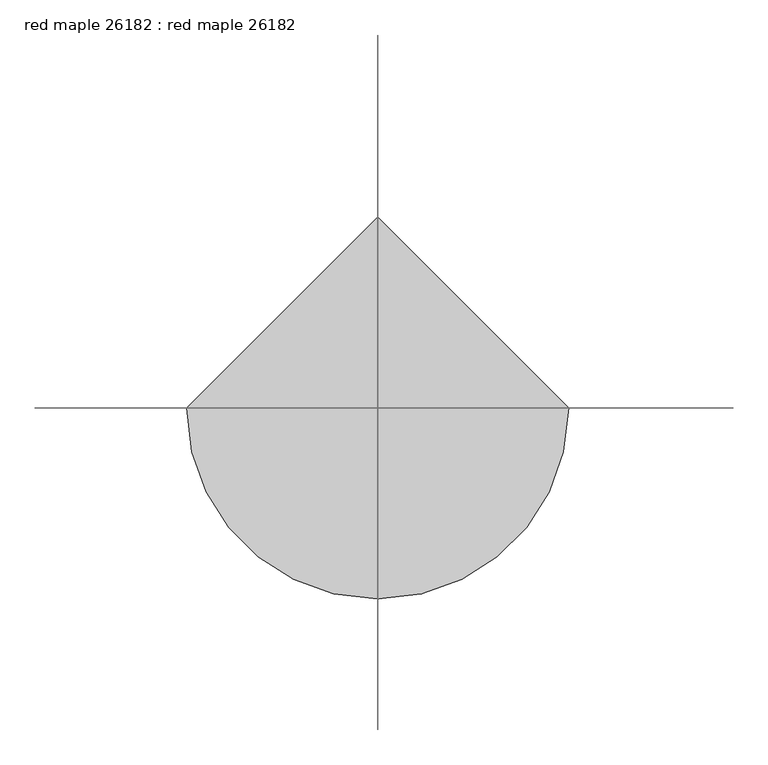
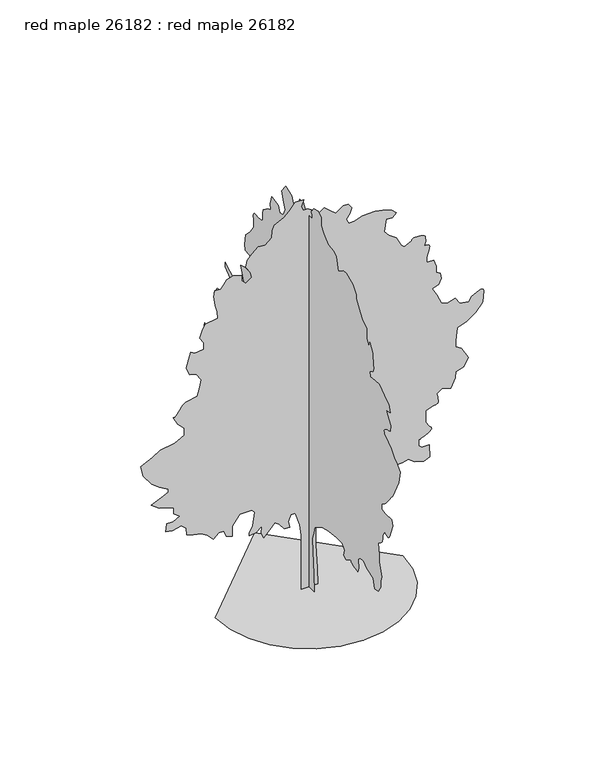
"""IFC4 building model written with IfcOpenShell, lengths in millimetres: proxy geometry, red maple 26182 : red maple 26182."""

from ifc_helpers import new_model, si_unit, origin, place, context, project, spatial, triangles, source, transform, mapped, element, save


def red_maple_26182_red_maple_26182_cba750cc(model_context):
    return source(origin(), model_context, "Body", "Tessellation", [
        triangles([(5.9e-06, 200.5240248, 0.0131599), (5.9e-06, -200.5423013, 0.0131599), (5.9e-06, -173.8047255, 401.079007), (5.9e-06, -147.0663684, 922.4677488), (5.9e-06, -133.6980892, 1216.5822092), (5.9e-06, -173.8047255, 1363.6407475), (5.9e-06, -227.2806583, 1537.4352264), (5.9e-06, -320.8632274, 1590.9124855), (5.9e-06, -534.7644153, 1711.2323215), (5.9e-06, -762.0361897, 1764.7071098), (5.9e-06, -1069.5212002, 1804.8136734), (5.9e-06, -1283.4223881, 1804.8136734), (5.9e-06, -1377.0037399, 1697.8617714), (5.9e-06, -1336.897031, 1550.8033058), (5.9e-06, -1443.848933, 1510.6967422), (5.9e-06, -1617.6460281, 1604.2805649), (5.9e-06, -1620.762553, 1592.8200726), (5.9e-06, -1625.400642, 1581.362051), (5.9e-06, -1633.0790977, 1569.9041748), (5.9e-06, -1645.319339, 1558.4436825), (5.9e-06, -1663.6378429, 1546.9856609), (5.9e-06, -1689.5560284, 1535.5251686), (5.9e-06, -1724.595314, 1524.0672924), (5.9e-06, -1761.1942429, 1514.1662979), (5.9e-06, -1791.4812023, 1507.0721088), (5.9e-06, -1816.5027855, 1502.3197826), (5.9e-06, -1837.3156139, 1499.4343483), (5.9e-06, -1854.971077, 1497.9534794), (5.9e-06, -1870.5234707, 1497.4074371), (5.9e-06, -1885.021859, 1497.3286629), (5.9e-06, -1911.7604885, 1590.9124855), (5.9e-06, -1898.3924091, 1791.445594), (5.9e-06, -1978.6056816, 1871.6588665), (5.9e-06, -2112.293597, 1885.0269459), (5.9e-06, -2219.245499, 1778.0750439), (5.9e-06, -2473.2533958, 1697.8617714), (5.9e-06, -2540.1036758, 1497.3286629), (5.9e-06, -2660.4236572, 1510.6967422), (5.9e-06, -2767.3575371, 1671.125758), (5.9e-06, -2767.3575371, 1804.8136734), (5.9e-06, -2794.1038696, 1911.7655754), (5.9e-06, -2700.5302208, 2219.2479698), (5.9e-06, -2700.5302208, 2393.0450649), (5.9e-06, -2673.7838882, 2660.4236572), (5.9e-06, -2676.8572472, 2660.5759735), (5.9e-06, -2681.2261665, 2661.668058), (5.9e-06, -2688.1603363, 2664.6399696), (5.9e-06, -2698.9553169, 2670.4056061), (5.9e-06, -2714.9066689, 2679.9053169), (5.9e-06, -2737.284082, 2694.1038689), (5.9e-06, -2767.3575371, 2713.8904518), (5.9e-06, -2796.66912, 2738.3761665), (5.9e-06, -2816.8623642, 2765.6558968), (5.9e-06, -2829.4607231, 2795.2721123), (5.9e-06, -2835.9629425, 2826.7681549), (5.9e-06, -2837.9189278, 2859.6612053), (5.9e-06, -2836.8265526, 2893.4940239), (5.9e-06, -2834.2104332, 2927.8096619), (5.9e-06, -2914.423851, 3061.4898743), (5.9e-06, -2945.8434448, 3041.8556076), (5.9e-06, -2976.6790627, 3024.6598549), (5.9e-06, -3006.3211487, 3012.3917084), (5.9e-06, -3034.2357239, 3007.4641022), (5.9e-06, -3059.8135231, 3012.3917084), (5.9e-06, -3082.4449905, 3029.5618813), (5.9e-06, -3101.5964378, 3061.4898743), (5.9e-06, -3235.2766502, 3382.3429642), (5.9e-06, -3195.1700867, 3516.0231766), (5.9e-06, -2941.1698929, 3502.6629456), (5.9e-06, -2794.1038696, 3516.0231766), (5.9e-06, -2807.4641006, 3649.7289688), (5.9e-06, -2841.8811859, 3670.0236603), (5.9e-06, -2876.5523254, 3691.8420959), (5.9e-06, -2911.6551247, 3716.7088921), (5.9e-06, -2947.4692177, 3746.1475021), (5.9e-06, -2984.2230789, 3781.6566719), (5.9e-06, -3022.1707626, 3824.7604362), (5.9e-06, -3061.4898743, 3876.98283), (5.9e-06, -3098.0914192, 3928.4433517), (5.9e-06, -3128.3680595, 3969.3626564), (5.9e-06, -3153.3871719, 4001.5191238), (5.9e-06, -3174.2152611, 4026.6652634), (5.9e-06, -3191.8682533, 4046.5280045), (5.9e-06, -3207.412944, 4062.9110161), (5.9e-06, -3221.9164192, 4077.5159386), (5.9e-06, -3449.1958603, 4532.0748207), (5.9e-06, -3516.0231766, 4826.1815781), (5.9e-06, -3368.9824425, 4986.6084137), (5.9e-06, -3302.1295464, 4999.9686447), (5.9e-06, -3155.0635231, 5187.1415222), (5.9e-06, -3061.4898743, 5253.9944183), (5.9e-06, -3024.5075386, 5271.2916183), (5.9e-06, -2989.023658, 5289.3004028), (5.9e-06, -2956.5878471, 5308.7056137), (5.9e-06, -2928.7238503, 5330.2194168), (5.9e-06, -2906.9559929, 5354.5528152), (5.9e-06, -2892.7574409, 5382.3656525), (5.9e-06, -2887.6775185, 5414.4206726), (5.9e-06, -2894.7134262, 5445.6629517), (5.9e-06, -2914.3474022, 5471.3166183), (5.9e-06, -2944.5228859, 5492.2973145), (5.9e-06, -2983.1054146, 5509.5183563), (5.9e-06, -3028.0125572, 5523.9453827), (5.9e-06, -3077.1107231, 5536.493454), (5.9e-06, -3128.3171906, 5548.100885), (5.9e-06, -3141.7030014, 5695.1669083), (5.9e-06, -3074.850396, 5802.1010788), (5.9e-06, -2967.8906456, 5949.1671021), (5.9e-06, -3128.3171906, 5989.2739563), (5.9e-06, -3074.850396, 6149.7007919), (5.9e-06, -2901.0633293, 6256.6599609), (5.9e-06, -2700.5302208, 6403.7009857), (5.9e-06, -2526.7306549, 6390.3401733), (5.9e-06, -2366.3039646, 6376.9799423), (5.9e-06, -2339.5653351, 6483.9141129), (5.9e-06, -2419.7786076, 6537.4061966), (5.9e-06, -2434.0052101, 6540.4798462), (5.9e-06, -2447.6476913, 6544.8487656), (5.9e-06, -2460.1190231, 6551.7826447), (5.9e-06, -2470.8378456, 6562.577916), (5.9e-06, -2479.217276, 6578.5292679), (5.9e-06, -2484.6730476, 6600.9063904), (5.9e-06, -2486.6238007, 6630.9801361), (5.9e-06, -2485.4529419, 6668.4702896), (5.9e-06, -2482.1813393, 6711.5746353), (5.9e-06, -2477.1522858, 6759.3769501), (5.9e-06, -2470.7209923, 6810.8883408), (5.9e-06, -2463.2380188, 6865.2193268), (5.9e-06, -2455.0515999, 6921.4292679), (5.9e-06, -2446.5172371, 6978.5792679), (5.9e-06, -2339.5653351, 7165.7521454), (5.9e-06, -2299.4587715, 7058.792395), (5.9e-06, -2232.6135784, 7179.1123764), (5.9e-06, -2232.6135784, 7433.1125702), (5.9e-06, -2058.8189541, 7540.0723206), (5.9e-06, -1938.499118, 7700.4985748), (5.9e-06, -1818.1791367, 7874.2856415), (5.9e-06, -1818.1791367, 7967.8845795), (5.9e-06, -1684.4887505, 8128.3114151), (5.9e-06, -1443.848933, 8248.6313965), (5.9e-06, -1310.1610176, 8221.8847733), (5.9e-06, -1136.3639225, 8101.5647919), (5.9e-06, -1042.7825706, 8395.6718399), (5.9e-06, -949.198748, 8462.524736), (5.9e-06, -735.2975601, 8489.2707779), (5.9e-06, -574.8710515, 8649.6976135), (5.9e-06, -467.9217293, 8770.0175949), (5.9e-06, -467.9217293, 8957.1648926), (5.9e-06, -347.6018206, 9037.3780197), (5.9e-06, -187.1730047, 8997.2711655), (5.9e-06, -93.5917073, 8876.9517654), (5.9e-06, -107.5840764, 8845.6589081), (5.9e-06, -119.5886307, 8815.6357407), (5.9e-06, -127.6175737, 8788.2036942), (5.9e-06, -129.6833633, 8764.6324585), (5.9e-06, -123.7979213, 8746.192305), (5.9e-06, -107.9734512, 8734.1779221), (5.9e-06, -80.2224107, 8729.9107407), (5.9e-06, 106.9427183, 8729.9107407), (5.9e-06, 227.262618, 8903.6978073), (5.9e-06, 360.9520595, 8890.3375763), (5.9e-06, 427.7947454, 8729.9107407), (5.9e-06, 601.5918769, 8649.6976135), (5.9e-06, 668.4345629, 8783.3778259), (5.9e-06, 895.7063009, 8876.9517654), (5.9e-06, 1042.7648392, 8676.4180756), (5.9e-06, 975.9195734, 8449.164505), (5.9e-06, 922.4449305, 8302.0984818), (5.9e-06, 989.2901236, 8141.6716461), (5.9e-06, 1122.9781116, 8114.9256042), (5.9e-06, 1176.4527546, 8261.9916275), (5.9e-06, 1443.8312016, 8288.7376694), (5.9e-06, 1497.3083153, 8101.5647919), (5.9e-06, 1470.5696857, 7967.8845795), (5.9e-06, 1590.8896671, 7927.7783066), (5.9e-06, 1764.6841461, 7794.0725143), (5.9e-06, 1778.0546963, 7700.4985748), (5.9e-06, 1778.0546963, 7540.0723206), (5.9e-06, 1844.8974186, 7499.9654663), (5.9e-06, 2005.3239635, 7499.9654663), (5.9e-06, 2036.5838287, 7505.2994431), (5.9e-06, 2066.3221298, 7508.2969345), (5.9e-06, 2093.0200642, 7506.6202927), (5.9e-06, 2115.1586838, 7497.9336136), (5.9e-06, 2131.2167152, 7479.8998306), (5.9e-06, 2139.6749199, 7450.1562973), (5.9e-06, 2139.0144951, 7406.3921082), (5.9e-06, 2134.0639252, 7358.3095779), (5.9e-06, 2130.5182114, 7316.5772415), (5.9e-06, 2128.1407402, 7280.1033051), (5.9e-06, 2126.6979504, 7247.8198105), (5.9e-06, 2125.9562805, 7218.7111221), (5.9e-06, 2125.6844948, 7191.6854462), (5.9e-06, 2125.6464157, 7165.7521454), (5.9e-06, 2259.3343311, 6978.5792679), (5.9e-06, 2433.1289555, 6804.7922012), (5.9e-06, 2473.2356644, 6550.767009), (5.9e-06, 2446.4995056, 6430.4470276), (5.9e-06, 2312.8089741, 6417.0867966), (5.9e-06, 2205.8596882, 6390.3401733), (5.9e-06, 2125.6464157, 6216.5531067), (5.9e-06, 2232.5957016, 6016.0199982), (5.9e-06, 2473.2356644, 6016.0199982), (5.9e-06, 2633.6520355, 5962.5279144), (5.9e-06, 2499.9741486, 5614.9537811), (5.9e-06, 2620.2915138, 5481.2479889), (5.9e-06, 2954.5048347, 5521.3548431), (5.9e-06, 3048.1040634, 5574.8475082), (5.9e-06, 3235.2513611, 5668.4208664), (5.9e-06, 3221.8908394, 5574.8475082), (5.9e-06, 2981.2511673, 5360.9280075), (5.9e-06, 2887.6775185, 5066.8215408), (5.9e-06, 2994.611689, 4839.5420998), (5.9e-06, 3141.6777122, 4852.9279106), (5.9e-06, 3144.9033875, 4867.1011734), (5.9e-06, 3150.3643913, 4880.4869843), (5.9e-06, 3160.2704727, 4892.2217331), (5.9e-06, 3176.8313805, 4901.4926788), (5.9e-06, 3202.2821526, 4907.4870804), (5.9e-06, 3238.8581177, 4909.3921967), (5.9e-06, 3288.7437355, 4906.3947052), (5.9e-06, 3529.3836983, 4879.6486633), (5.9e-06, 3649.703389, 4705.8618874), (5.9e-06, 3609.5968254, 4518.6890099), (5.9e-06, 3462.5308022, 4411.7548393), (5.9e-06, 3342.2108208, 4117.6227928), (5.9e-06, 3395.677906, 3930.4752045), (5.9e-06, 3449.1702805, 3863.622599), (5.9e-06, 3582.8507835, 3636.343158), (5.9e-06, 3850.2367882, 3663.0891998), (5.9e-06, 4024.0235641, 3770.0489502), (5.9e-06, 4077.4906494, 3529.4089874), (5.9e-06, 3823.4904556, 3409.089006), (5.9e-06, 3649.703389, 3355.5966316), (5.9e-06, 3529.3836983, 3088.2362068), (5.9e-06, 3462.5308022, 2927.8096619), (5.9e-06, 3382.3173843, 2700.5302208), (5.9e-06, 3235.2513611, 2727.2762627), (5.9e-06, 3007.9974998, 2767.3831169), (5.9e-06, 2820.8246223, 2727.2762627), (5.9e-06, 2687.1444099, 2513.364901), (5.9e-06, 2860.9311859, 2339.570422), (5.9e-06, 3021.3577309, 2312.8319378), (5.9e-06, 3048.1040634, 2058.8215702), (5.9e-06, 3036.4454727, 2033.2918785), (5.9e-06, 3023.6183487, 2009.2838963), (5.9e-06, 3008.4547394, 1988.3135193), (5.9e-06, 2989.7855301, 1971.9052185), (5.9e-06, 2966.4430595, 1961.5775059), (5.9e-06, 2937.258213, 1958.8496201), (5.9e-06, 2901.0380402, 1965.2402184), (5.9e-06, 2863.2679619, 1977.8690987), (5.9e-06, 2829.7147774, 1992.6010483), (5.9e-06, 2799.6663208, 2009.0882687), (5.9e-06, 2772.4121704, 2026.9800545), (5.9e-06, 2747.2916107, 2045.9209042), (5.9e-06, 2723.5424789, 2065.5651993), (5.9e-06, 2700.504641, 2085.5600544), (5.9e-06, 2606.9309921, 2192.5119564), (5.9e-06, 2589.5829231, 2220.7695339), (5.9e-06, 2571.2947952, 2246.6877193), (5.9e-06, 2551.1527107, 2267.9297367), (5.9e-06, 2528.193647, 2282.1561939), (5.9e-06, 2501.4929512, 2287.0279896), (5.9e-06, 2470.1189941, 2280.208057), (5.9e-06, 2433.1289555, 2259.3571495), (5.9e-06, 2386.7865807, 2232.2681053), (5.9e-06, 2329.2174202, 2207.9857212), (5.9e-06, 2262.2959236, 2186.0425838), (5.9e-06, 2187.8891281, 2165.9689545), (5.9e-06, 2107.8714832, 2147.2998905), (5.9e-06, 2024.1123516, 2129.5656532), (5.9e-06, 1938.4812412, 2112.2986839), (5.9e-06, 1724.5775826, 2058.8215702), (5.9e-06, 1791.4227757, 1925.1335094), (5.9e-06, 2005.3239635, 1791.445594), (5.9e-06, 2112.2758656, 1617.6484989), (5.9e-06, 1925.1106911, 1550.8033058), (5.9e-06, 1899.2305847, 1550.9989334), (5.9e-06, 1872.766357, 1552.362949), (5.9e-06, 1845.1311253, 1556.0662113), (5.9e-06, 1815.7433842, 1563.2772537), (5.9e-06, 1784.0161057, 1575.1644642), (5.9e-06, 1749.3654591, 1592.8988468), (5.9e-06, 1711.2095032, 1617.6484989), (5.9e-06, 1671.8826885, 1646.6858253), (5.9e-06, 1633.9579685, 1676.4242718), (5.9e-06, 1597.2041073, 1706.7493103), (5.9e-06, 1561.3849274, 1737.539146), (5.9e-06, 1526.2668674, 1768.6821579), (5.9e-06, 1491.6162209, 1800.0587311), (5.9e-06, 1457.1991356, 1831.5523029), (5.9e-06, 1189.8233047, 1911.7655754), (5.9e-06, 975.9195734, 1951.872139), (5.9e-06, 762.0183855, 2005.3467819), (5.9e-06, 548.1146542, 1965.2402184), (5.9e-06, 253.9999576, 1858.2883163), (5.9e-06, 173.7866851, 1751.3390305), (5.9e-06, 106.9427183, 1564.173856), (5.9e-06, 80.2041161, 1296.7955544), (5.9e-06, 106.9427183, 935.8358282), (5.9e-06, 160.4173885, 414.4495934), (-2085.2019367, 0.0, 0.0), (-2030.0762318, -477.7896226, 0.0), (-1873.078838, -916.5648388, 0.0), (-1626.7799183, -1303.7500717, 0.0), (-1303.7500717, -1626.7799183, 0.0), (-916.5648388, -1873.078838, 0.0), (-477.7896226, -2030.0762318, 0.0), (9.11e-05, -2085.2019367, 0.0), (477.7896226, -2030.0762318, 0.0), (916.5648388, -1873.078838, 0.0), (1303.7500717, -1626.7799183, 0.0), (1626.7799183, -1303.7500717, 0.0), (1873.078838, -916.5648388, 0.0), (2030.0762318, -477.7896226, 0.0), (2085.2019367, 0.0001828, 0.0), (-0.0002734, 2085.2019367, 0.0), (199.8874902, 0.0002285, 0.005264), (-169.704903, 0.0002285, 0.005264), (-169.704903, 0.0001919, 684.4365658), (-169.704903, 0.0001645, 1040.3416586), (-169.704903, 0.0001554, 1273.0464226), (-210.770892, 0.0001371, 1533.1325821), (-306.5909517, 0.0001188, 1834.2801888), (-402.4125375, 0.0001188, 1834.2801888), (-457.1673348, 0.0001279, 1683.7063854), (-429.7886644, 0.0001371, 1546.8205547), (-552.9863771, 0.0001371, 1560.5086727), (-662.4960445, 0.0001279, 1697.3945034), (-758.317594, 0.0001279, 1765.8374187), (-867.8247179, 0.0001279, 1642.639706), (-1004.7104759, 0.0001371, 1505.7538754), (-1059.465346, 0.0001371, 1628.9515881), (-1045.777228, 0.0001279, 1793.2159801), (-1182.6630587, 0.0001279, 1683.7063854), (-1333.2394054, 0.0001279, 1670.0182674), (-1333.2394054, 0.0001279, 1738.4611828), (-1251.1059013, 0.0001188, 1875.3470135), (-1210.0416927, 0.0001005, 2176.4972363), (-1278.4846081, 0.0001005, 2244.9401516), (-1538.5681515, 0.0001005, 2244.9401516), (-1702.8300728, 0.0001097, 2012.2328442), (-1702.8300728, 0.0001188, 1916.4136929), (-1702.8300728, 0.0001279, 1779.5280075), (-1839.7183743, 0.0001188, 1834.2801888), (-1894.4731716, 0.0001097, 1971.1686356), (-2003.9802956, 0.0001097, 1971.1686356), (-2127.1780083, 0.0001188, 1861.6588955), (-2264.063839, 0.0001097, 1998.5447262), (-2400.9521404, 0.0001097, 2080.6756142), (-2578.9149696, 0.0001005, 2121.7424389), (-2715.7955681, 0.0001005, 2176.4972363), (-2729.4863022, 9.14e-05, 2327.0711849), (-2838.9857231, 8.22e-05, 2422.8926617), (-3044.3194107, 9.14e-05, 2381.8259823), (-3181.2000092, 8.22e-05, 2409.204689), (-3167.5095657, 7.31e-05, 2587.1444092), (-3016.9382332, 7.31e-05, 2587.1444092), (-2880.0576347, 7.31e-05, 2669.2882324), (-3003.2474991, 6.4e-05, 2765.0969193), (-3003.2474991, 5.48e-05, 2902.0030975), (-3140.1283882, 5.48e-05, 2956.7401634), (-3331.7713417, 5.48e-05, 3011.5025185), (-3509.7241425, 4.57e-05, 3148.3834076), (-3290.6997208, 3.66e-05, 3244.2176743), (-3126.4376541, 3.66e-05, 3312.6451836), (-3126.4376541, 2.74e-05, 3381.0982727), (-3331.7713417, 1.83e-05, 3504.2884277), (-3496.0334084, 1.83e-05, 3627.5038719), (-3687.6766525, 0.0, 3887.5746254), (-3742.4390076, -1.83e-05, 4133.9802246), (-3632.9395866, -1.83e-05, 4188.7172905), (-3482.3426743, -2.74e-05, 4257.1703796), (-3304.3901642, -2.74e-05, 4366.6698006), (-2989.5570557, -3.66e-05, 4421.4324463), (-2770.532634, -3.66e-05, 4530.9318672), (-2770.532634, -4.57e-05, 4695.1936432), (-2921.1292557, -5.48e-05, 4845.7905556), (-3016.9382332, -7.31e-05, 5023.742775), (-3007.9974998, -7.31e-05, 5021.1266556), (-2998.2184456, -7.31e-05, 5020.5679688), (-2986.7630402, -7.31e-05, 5024.0985672), (-2972.7929626, -7.31e-05, 5033.6997253), (-2955.4701828, -7.31e-05, 5051.4544556), (-2933.9816689, -7.31e-05, 5079.3946106), (-2907.4388123, -7.31e-05, 5119.5520432), (-2879.295472, -7.31e-05, 5162.0971207), (-2853.3113022, -8.22e-05, 5196.7426804), (-2829.1305107, -8.22e-05, 5224.783992), (-2806.3720161, -8.22e-05, 5247.5680664), (-2784.7058968, -8.22e-05, 5266.4145905), (-2763.7507805, -8.22e-05, 5282.6199966), (-2743.1767456, -8.22e-05, 5297.5045532), (-2483.0830284, -9.14e-05, 5352.2669083), (-2428.328231, -0.0001005, 5543.9098618), (-2400.9521404, -0.0001097, 5708.1719284), (-2510.4618805, -0.0001188, 5872.4339951), (-2647.3424789, -0.0001188, 5913.4803268), (-2729.4863022, -0.0001371, 6091.4328369), (-2674.7236565, -0.0001462, 6283.0757904), (-2633.6520355, -0.0001554, 6433.6474136), (-2537.8378258, -0.0001462, 6378.9100571), (-2346.1973431, -0.0001554, 6406.2915253), (-2346.1973431, -0.0001645, 6556.8625671), (-2428.328231, -0.0001645, 6693.7437469), (-2373.5734337, -0.0001736, 6844.3147888), (-2305.1305183, -0.0001828, 6981.1953873), (-2031.3590023, -0.0001919, 7022.2672989), (-2045.0471203, -0.0002011, 7186.5293655), (-2086.1137997, -0.0002102, 7337.1004074), (-2113.4900356, -0.0002193, 7556.1248291), (-2099.8019176, -0.0002285, 7693.0060089), (-1962.916087, -0.0002285, 7679.3149841), (-1894.4731716, -0.0002285, 7761.4588074), (-1826.0302563, -0.0002376, 7857.2674942), (-1689.1419548, -0.0002376, 7898.3394058), (-1497.5013268, -0.0002376, 7843.5770508), (-1497.5013268, -0.0002285, 7720.3868958), (-1401.6823208, -0.0002285, 7624.5782089), (-1278.4846081, -0.0002285, 7720.3868958), (-1305.8606987, -0.0002376, 7857.2674942), (-1401.6823208, -0.0002467, 8007.8391174), (-1374.303614, -0.0002559, 8158.4357391), (-1264.7940193, -0.000265, 8267.9354507), (-1127.9081886, -0.0002742, 8391.1250244), (-977.3343853, -0.000265, 8377.434581), (-826.7605093, -0.0002742, 8500.6503159), (-813.0699205, -0.0002833, 8651.2213577), (-772.0057119, -0.0002924, 8774.4115128), (-566.6744588, -0.0003016, 8870.2457794), (-443.4767461, -0.0003016, 8979.745491), (-306.5909517, -0.0003107, 9144.0075577), (-114.9505871, -0.0003107, 9144.0075577), (-169.704903, -0.0003016, 8993.4359344), (-128.6391684, -0.0003016, 8897.6016678), (-32.8188589, -0.0003016, 8897.6016678), (49.3128694, -0.0002924, 8842.8648926), (76.6900319, -0.0002924, 8733.3396011), (240.9532249, -0.0002924, 8719.6491577), (336.7737751, -0.0002924, 8788.1019562), (473.6595695, -0.0002833, 8678.6028259), (596.8572822, -0.0002833, 8569.0781158), (761.1217833, -0.0002833, 8692.2932693), (870.6314507, -0.0002833, 8692.2932693), (952.7624113, -0.0002833, 8582.7685593), (911.6956593, -0.0002742, 8445.8879608), (829.5646986, -0.000265, 8350.0786926), (884.319496, -0.000265, 8240.5539825), (1007.5172087, -0.000265, 8240.5539825), (1199.1578367, -0.000265, 8309.006781), (1472.9294254, -0.000265, 8309.006781), (1637.1938175, -0.000265, 8281.6258942), (1842.5225636, -0.0002559, 8213.1725143), (1938.3441856, -0.0002559, 8117.3638275), (1856.2106815, -0.0002467, 8021.5295609), (1719.3248508, -0.0002467, 8035.2200043), (1691.9487602, -0.0002376, 7912.0298492), (1678.2580261, -0.0002285, 7761.4588074), (1774.0796482, -0.0002285, 7638.2686523), (1938.3441856, -0.0002193, 7528.7439423), (2047.8513096, -0.0002011, 7309.7195206), (2116.2940796, -0.0002011, 7254.982164), (2280.558617, -0.0002102, 7337.1004074), (2283.7919952, -0.0002102, 7348.7589981), (2288.8187233, -0.0002102, 7359.9350601), (2297.439418, -0.0002102, 7370.1460648), (2311.4475746, -0.0002102, 7378.9344818), (2332.6388683, -0.0002102, 7385.7927841), (2362.8089745, -0.0002102, 7390.2628601), (2403.7563297, -0.0002102, 7391.8633438), (2446.2989365, -0.0002102, 7390.2628601), (2480.9392639, -0.0002102, 7385.7927841), (2508.9962723, -0.0002102, 7378.9344818), (2531.7826721, -0.0002102, 7370.1460648), (2550.619313, -0.0002102, 7359.9350601), (2566.8244286, -0.0002102, 7348.7589981), (2581.7089851, -0.0002102, 7337.1004074), (2595.3994286, -0.0002011, 7213.9108337), (2568.018251, -0.0001919, 7118.1015656), (2599.8953751, -0.0001919, 7117.6446167), (2629.5115906, -0.0001919, 7114.5709671), (2654.581572, -0.0001919, 7106.2400803), (2672.8188309, -0.0001919, 7089.9840958), (2681.9627495, -0.0001919, 7063.2124741), (2679.7274208, -0.0001919, 7023.2579361), (2663.8525177, -0.0001828, 6967.5049438), (2643.9641968, -0.0001828, 6908.5771454), (2630.5530968, -0.0001828, 6859.6818741), (2622.5268425, -0.0001736, 6819.1686493), (2618.8183479, -0.0001736, 6785.3614105), (2618.3358192, -0.0001736, 6756.6085144), (2620.0121704, -0.0001736, 6731.1833221), (2622.7806061, -0.0001736, 6707.4341904), (2773.3519386, -0.0001736, 6707.4341904), (2828.1145844, -0.0001554, 6543.1721237), (2828.1145844, -0.0001554, 6406.2915253), (2923.9232712, -0.0001462, 6351.5291702), (2937.6140053, -0.0001371, 6228.3390152), (2882.8516502, -0.0001371, 6105.1232803), (2745.9707611, -0.0001279, 6050.3865051), (2841.8050278, -0.0001188, 5872.4339951), (2937.6140053, -0.0001097, 5653.4095734), (3074.4946037, -0.0001005, 5584.9561935), (3252.4471138, -0.0001097, 5639.7191299), (3348.2813805, -0.0001005, 5489.1475067), (3553.5897789, -9.14e-05, 5461.7666199), (3622.042868, -0.0001005, 5557.5753067), (3677.3894897, -0.0001005, 5589.3251129), (3730.4754936, -0.0001005, 5617.7989563), (3779.0149727, -0.0001097, 5639.8458664), (3820.6964401, -0.0001097, 5652.1648819), (3853.3101471, -0.0001097, 5651.5806152), (3874.5446068, -0.0001097, 5634.8165222), (3882.1392014, -0.0001005, 5598.6472183), (3881.3261696, -0.0001005, 5553.3081253), (3879.0911316, -0.0001005, 5510.8647858), (3875.6619804, -9.14e-05, 5470.7835114), (3871.2677719, -9.14e-05, 5432.6323517), (3866.1625603, -9.14e-05, 5395.9293594), (3860.5745293, -9.14e-05, 5360.1664261), (3854.7580238, -9.14e-05, 5324.8854401), (3704.1866913, -7.31e-05, 5160.6239548), (3512.5434471, -6.4e-05, 5010.0523315), (3293.5190254, -6.4e-05, 4941.5995331), (3266.1378479, -4.57e-05, 4640.4565773), (3266.1378479, -3.66e-05, 4503.5506897), (3389.3280029, -3.66e-05, 4421.4324463), (3539.9246246, -1.83e-05, 4161.336113), (3444.090358, -9.1e-06, 3969.7184486), (3266.1378479, 0.0, 3914.9558029), (3252.4471138, 9.1e-06, 3778.0752045), (3156.638427, 1.83e-05, 3559.0507828), (2964.9951828, 1.83e-05, 3627.5038719), (2846.3771324, 1.83e-05, 3536.8765549), (2845.4879425, 1.83e-05, 3538.3244316), (2845.1071518, 1.83e-05, 3537.5369797), (2845.7675766, 1.83e-05, 3532.3047409), (2847.9773254, 1.83e-05, 3520.3665161), (2852.269796, 1.83e-05, 3499.5131378), (2859.1786766, 2.74e-05, 3467.5345665), (2869.1609161, 2.74e-05, 3422.1701843), (2875.307634, 2.74e-05, 3376.1453773), (2871.3959541, 2.74e-05, 3342.3378479), (2859.1025185, 3.66e-05, 3318.7157433), (2840.1286766, 3.66e-05, 3303.2219215), (2816.1002014, 3.66e-05, 3293.8492378), (2788.7190239, 3.66e-05, 3288.5405502), (2759.6614952, 3.66e-05, 3285.264006), (2595.3994286, 3.66e-05, 3230.5269402), (2595.3994286, 5.48e-05, 2956.7401634), (2677.517672, 6.4e-05, 2833.5500084), (2697.53302, 6.4e-05, 2815.871727), (2714.297113, 6.4e-05, 2797.7106262), (2724.5839851, 6.4e-05, 2778.5844681), (2725.1682518, 6.4e-05, 2758.0357224), (2712.8492363, 6.4e-05, 2735.582151), (2684.3503944, 7.31e-05, 2710.7156456), (2636.4713402, 7.31e-05, 2682.9786758), (2584.1727882, 7.31e-05, 2657.2229805), (2543.4055092, 7.31e-05, 2637.9697952), (2512.1864845, 7.31e-05, 2624.0761665), (2488.640538, 7.31e-05, 2614.5002975), (2470.8427872, 7.31e-05, 2608.1503944), (2456.8753258, 7.31e-05, 2603.9593712), (2444.8231544, 7.31e-05, 2600.8351433), (2444.8231544, 8.22e-05, 2463.9594864), (2513.2660698, 9.14e-05, 2395.5139549), (2677.517672, 9.14e-05, 2395.5139549), (2691.2084061, 0.0001005, 2108.0543209), (2554.3275169, 0.0001097, 2053.2995235), (2349.0015324, 0.0001005, 2121.7424389), (2212.1157017, 0.0001005, 2217.564061), (2075.229871, 0.0001005, 2190.1853542), (1828.8344456, 0.0001005, 2176.4972363), (1678.2580261, 0.0001005, 2135.4305569), (1664.5700535, 0.0001188, 1943.7899288), (1513.9961048, 0.0001188, 1930.1018108), (1322.3554768, 0.0001188, 1943.7899288), (1240.2219727, 0.0001188, 1820.5922161), (952.7624113, 0.0001279, 1779.5280075), (733.7430765, 0.0001188, 1834.2801888), (733.7430765, 0.0001371, 1615.2634701), (555.7930736, 0.0001371, 1628.9515881), (501.0382762, 0.0001279, 1738.4611828), (405.2166904, 0.0001279, 1697.3945034), (295.7070412, 0.0001279, 1697.3945034), (254.6428326, 0.0001188, 1820.5922161), (145.13292, 0.0001279, 1697.3945034), (131.4443387, 0.0001371, 1546.8205547), (145.13292, 0.0001554, 1314.1132473), (145.13292, 0.0001736, 930.8319912), (186.1989181, 0.0002102, 383.2863067)], [[130, 131, 132], [208, 209, 210], [208, 210, 211], [207, 208, 211], [230, 231, 232], [230, 232, 233], [276, 277, 278], [229, 230, 233], [229, 233, 234], [302, 1, 2], [302, 2, 3], [302, 3, 4], [301, 302, 4], [301, 4, 5], [300, 301, 5], [300, 5, 6], [299, 300, 6], [299, 6, 7], [108, 109, 110], [203, 204, 205], [206, 207, 211], [206, 211, 212], [108, 110, 111], [202, 203, 205], [13, 14, 15], [13, 15, 16], [236, 237, 238], [171, 172, 173], [170, 171, 173], [170, 173, 174], [36, 37, 38], [36, 38, 39], [36, 39, 40], [275, 276, 278], [275, 278, 279], [275, 279, 280], [275, 280, 281], [275, 281, 282], [275, 282, 283], [275, 283, 284], [275, 284, 285], [275, 285, 286], [275, 286, 287], [275, 287, 288], [275, 288, 289], [275, 289, 290], [274, 275, 290], [274, 290, 291], [274, 291, 292], [67, 68, 69], [66, 67, 69], [164, 165, 166], [164, 166, 167], [163, 164, 167], [163, 167, 168], [242, 243, 244], [29, 30, 31], [104, 105, 106], [197, 198, 199], [28, 29, 31], [298, 299, 7], [66, 69, 70], [65, 66, 70], [64, 65, 70], [63, 64, 70], [62, 63, 70], [61, 62, 70], [60, 61, 70], [59, 60, 70], [27, 28, 31], [150, 151, 152], [160, 161, 162], [159, 160, 162], [196, 197, 199], [195, 196, 199], [195, 199, 200], [26, 27, 31], [133, 134, 135], [242, 244, 245], [242, 245, 246], [242, 246, 247], [242, 247, 248], [242, 248, 249], [242, 249, 250], [242, 250, 251], [242, 251, 252], [242, 252, 253], [242, 253, 254], [242, 254, 255], [242, 255, 256], [242, 256, 257], [242, 257, 258], [242, 258, 259], [241, 242, 259], [241, 259, 260], [241, 260, 261], [241, 261, 262], [241, 262, 263], [241, 263, 264], [298, 7, 8], [274, 292, 293], [147, 148, 149], [147, 149, 150], [147, 150, 152], [147, 152, 153], [147, 153, 154], [147, 154, 155], [147, 155, 156], [36, 40, 41], [36, 41, 42], [35, 36, 42], [34, 35, 42], [34, 42, 43], [86, 87, 88], [86, 88, 89], [34, 43, 44], [104, 106, 107], [103, 104, 107], [102, 103, 107], [25, 26, 31], [25, 31, 32], [24, 25, 32], [23, 24, 32], [22, 23, 32], [21, 22, 32], [20, 21, 32], [19, 20, 32], [18, 19, 32], [17, 18, 32], [16, 17, 32], [13, 16, 32], [12, 13, 32], [102, 107, 108], [101, 102, 108], [129, 130, 132], [146, 147, 156], [100, 101, 108], [236, 238, 239], [146, 156, 157], [221, 222, 223], [221, 223, 224], [221, 224, 225], [220, 221, 225], [219, 220, 225], [218, 219, 225], [217, 218, 225], [216, 217, 225], [215, 216, 225], [214, 215, 225], [213, 214, 225], [213, 225, 226], [33, 34, 44], [235, 236, 239], [298, 8, 9], [297, 298, 9], [12, 32, 33], [58, 59, 70], [175, 176, 177], [85, 86, 89], [85, 89, 90], [85, 90, 91], [85, 91, 92], [84, 85, 92], [84, 92, 93], [83, 84, 93], [82, 83, 93], [82, 93, 94], [81, 82, 94], [80, 81, 94], [80, 94, 95], [79, 80, 95], [12, 33, 44], [78, 79, 95], [77, 78, 95], [76, 77, 95], [75, 76, 95], [74, 75, 95], [73, 74, 95], [72, 73, 95], [71, 72, 95], [71, 95, 96], [108, 111, 112], [108, 112, 113], [100, 108, 113], [100, 113, 114], [99, 100, 114], [98, 99, 114], [194, 195, 200], [128, 129, 132], [137, 138, 139], [175, 177, 178], [174, 175, 178], [241, 264, 265], [139, 140, 141], [139, 141, 142], [137, 139, 142], [229, 234, 235], [229, 235, 239], [228, 229, 239], [227, 228, 239], [227, 239, 240], [226, 227, 240], [213, 226, 240], [136, 137, 142], [142, 143, 144], [142, 144, 145], [145, 146, 157], [127, 128, 132], [11, 12, 44], [170, 174, 178], [194, 200, 201], [71, 96, 97], [145, 157, 158], [169, 170, 178], [212, 213, 240], [206, 212, 240], [205, 206, 240], [205, 240, 241], [205, 241, 265], [205, 265, 266], [205, 266, 267], [205, 267, 268], [205, 268, 269], [205, 269, 270], [205, 270, 271], [205, 271, 272], [205, 272, 273], [205, 273, 274], [205, 274, 293], [205, 293, 294], [205, 294, 295], [202, 205, 295], [202, 295, 296], [201, 202, 296], [201, 296, 297], [201, 297, 9], [201, 9, 10], [201, 10, 11], [201, 11, 44], [194, 201, 44], [193, 194, 44], [193, 44, 45], [193, 45, 46], [193, 46, 47], [193, 47, 48], [193, 48, 49], [193, 49, 50], [193, 50, 51], [193, 51, 52], [193, 52, 53], [193, 53, 54], [193, 54, 55], [193, 55, 56], [193, 56, 57], [193, 57, 58], [193, 58, 70], [193, 70, 71], [193, 71, 97], [193, 97, 98], [193, 98, 114], [193, 114, 115], [192, 193, 115], [191, 192, 115], [190, 191, 115], [189, 190, 115], [188, 189, 115], [187, 188, 115], [186, 187, 115], [185, 186, 115], [184, 185, 115], [183, 184, 115], [182, 183, 115], [181, 182, 115], [180, 181, 115], [179, 180, 115], [178, 179, 115], [169, 178, 115], [168, 169, 115], [163, 168, 115], [162, 163, 115], [159, 162, 115], [158, 159, 115], [145, 158, 115], [142, 145, 115], [136, 142, 115], [135, 136, 115], [133, 135, 115], [132, 133, 115], [127, 132, 115], [126, 127, 115], [126, 115, 116], [125, 126, 116], [124, 125, 116], [123, 124, 116], [122, 123, 116], [121, 122, 116], [121, 116, 117], [120, 121, 117], [120, 117, 118], [119, 120, 118], [317, 318, 303], [316, 317, 303], [316, 303, 304], [315, 316, 304], [315, 304, 305], [315, 305, 306], [314, 315, 306], [313, 314, 306], [313, 306, 307], [313, 307, 308], [313, 308, 309], [313, 309, 310], [313, 310, 311], [313, 311, 312], [379, 380, 381], [379, 381, 382], [364, 365, 366], [344, 345, 346], [332, 333, 334], [433, 434, 435], [327, 328, 329], [401, 402, 403], [327, 329, 330], [344, 346, 347], [343, 344, 347], [332, 334, 335], [432, 433, 435], [379, 382, 383], [534, 535, 536], [336, 337, 338], [336, 338, 339], [335, 336, 339], [582, 583, 584], [582, 584, 585], [593, 319, 320], [593, 320, 321], [592, 593, 321], [592, 321, 322], [591, 592, 322], [591, 322, 323], [412, 413, 414], [331, 332, 335], [591, 323, 324], [590, 591, 324], [568, 569, 570], [568, 570, 571], [568, 571, 572], [568, 572, 573], [567, 568, 573], [348, 349, 350], [532, 533, 534], [454, 455, 456], [454, 456, 457], [453, 454, 457], [357, 358, 359], [356, 357, 359], [355, 356, 359], [355, 359, 360], [363, 364, 366], [363, 366, 367], [589, 590, 324], [589, 324, 325], [576, 577, 578], [371, 372, 373], [335, 339, 340], [379, 383, 384], [504, 505, 506], [440, 441, 442], [417, 418, 419], [326, 327, 330], [494, 495, 496], [586, 587, 588], [362, 363, 367], [432, 435, 436], [588, 589, 325], [326, 330, 331], [352, 353, 354], [585, 586, 588], [452, 453, 457], [331, 335, 340], [379, 384, 385], [416, 417, 419], [415, 416, 419], [411, 412, 414], [531, 532, 534], [528, 529, 530], [528, 530, 531], [527, 528, 531], [431, 432, 436], [414, 415, 419], [411, 414, 419], [411, 419, 420], [410, 411, 420], [409, 410, 420], [576, 578, 579], [371, 373, 374], [370, 371, 374], [370, 374, 375], [369, 370, 375], [369, 375, 376], [368, 369, 376], [368, 376, 377], [407, 408, 409], [452, 457, 458], [451, 452, 458], [450, 451, 458], [450, 458, 459], [497, 498, 499], [497, 499, 500], [497, 500, 501], [445, 446, 447], [444, 445, 447], [443, 444, 447], [443, 447, 448], [326, 331, 340], [360, 361, 362], [494, 496, 497], [405, 406, 407], [405, 407, 409], [398, 399, 400], [398, 400, 401], [398, 401, 403], [398, 403, 404], [397, 398, 404], [579, 580, 581], [494, 497, 501], [425, 426, 427], [379, 385, 386], [429, 430, 431], [527, 531, 534], [477, 478, 479], [476, 477, 479], [475, 476, 479], [474, 475, 479], [473, 474, 479], [473, 479, 480], [472, 473, 480], [471, 472, 480], [470, 471, 480], [469, 470, 480], [468, 469, 480], [467, 468, 480], [466, 467, 480], [465, 466, 480], [464, 465, 480], [463, 464, 480], [566, 567, 573], [566, 573, 574], [566, 574, 575], [428, 429, 431], [428, 431, 436], [422, 423, 424], [422, 424, 425], [422, 425, 427], [421, 422, 427], [342, 343, 347], [437, 438, 439], [436, 437, 439], [428, 436, 439], [378, 379, 386], [378, 386, 387], [378, 387, 388], [378, 388, 389], [378, 389, 390], [378, 390, 391], [378, 391, 392], [378, 392, 393], [378, 393, 394], [378, 394, 395], [582, 585, 588], [351, 352, 354], [513, 514, 515], [512, 513, 515], [511, 512, 515], [511, 515, 516], [510, 511, 516], [510, 516, 517], [509, 510, 517], [509, 517, 518], [509, 518, 519], [508, 509, 519], [507, 508, 519], [507, 519, 520], [507, 520, 521], [507, 521, 522], [507, 522, 523], [507, 523, 524], [506, 507, 524], [506, 524, 525], [504, 506, 525], [503, 504, 525], [354, 355, 360], [579, 581, 582], [342, 347, 348], [342, 348, 350], [342, 350, 351], [342, 351, 354], [342, 354, 360], [342, 360, 362], [342, 362, 367], [342, 367, 368], [342, 368, 377], [341, 342, 377], [449, 450, 459], [527, 534, 536], [404, 405, 409], [341, 377, 378], [341, 378, 395], [341, 395, 396], [503, 525, 526], [440, 442, 443], [555, 556, 557], [554, 555, 557], [554, 557, 558], [553, 554, 558], [552, 553, 558], [552, 558, 559], [551, 552, 559], [551, 559, 560], [551, 560, 561], [551, 561, 562], [551, 562, 563], [551, 563, 564], [551, 564, 565], [551, 565, 566], [551, 566, 575], [550, 551, 575], [550, 575, 576], [460, 461, 462], [483, 484, 485], [482, 483, 485], [482, 485, 486], [481, 482, 486], [481, 486, 487], [480, 481, 487], [480, 487, 488], [463, 480, 488], [463, 488, 489], [463, 489, 490], [463, 490, 491], [463, 491, 492], [463, 492, 493], [463, 493, 494], [463, 494, 501], [341, 396, 397], [340, 341, 397], [326, 340, 397], [325, 326, 397], [588, 325, 397], [582, 588, 397], [579, 582, 397], [576, 579, 397], [550, 576, 397], [550, 397, 404], [550, 404, 409], [550, 409, 420], [550, 420, 421], [549, 550, 421], [549, 421, 427], [549, 427, 428], [549, 428, 439], [549, 439, 440], [549, 440, 443], [549, 443, 448], [549, 448, 449], [549, 449, 459], [549, 459, 460], [549, 460, 462], [549, 462, 463], [549, 463, 501], [549, 501, 502], [549, 502, 503], [548, 549, 503], [547, 548, 503], [526, 527, 536], [503, 526, 536], [544, 545, 546], [543, 544, 546], [543, 546, 547], [542, 543, 547], [541, 542, 547], [540, 541, 547], [503, 536, 537], [547, 503, 537], [547, 537, 538], [547, 538, 539], [540, 547, 539]], closed=False),
    ])


if __name__ == "__main__":
    model = new_model("IFC4")
    model_context = context("Model", 3, world=origin())
    ifc_project = project(units=[si_unit("LENGTHUNIT", "METRE", prefix="MILLI")], contexts=[model_context])
    site = spatial("IfcSite", under=ifc_project)
    building = spatial("IfcBuilding", under=site)
    placement = place(None, origin())
    red_maple_26182_red_maple_26182_shape = red_maple_26182_red_maple_26182_cba750cc(model_context)
    element("IfcBuildingElementProxy", 1, Name="red maple 26182 : red maple 26182", ObjectType="red maple 26182 : red maple 26182", at=placement, inside=building, context=model_context, shape_type="MappedRepresentation", body=[
        mapped(red_maple_26182_red_maple_26182_shape, transform((0.0, 0.0, 0.0), x_axis=(1.0, 0.0, 0.0), y_axis=(0.0, 1.0, 0.0), z_axis=(0.0, 0.0, 1.0))),
    ])
    save(model, "model.ifc")

# Revit data of these elements
# Type "red maple 26182 : red maple 26182"
#   built-in parameter 1005195 = "RPC-16-G0SR-83PX-Q347-6000-ST1L-LVER-AU"
#   Height = 0
